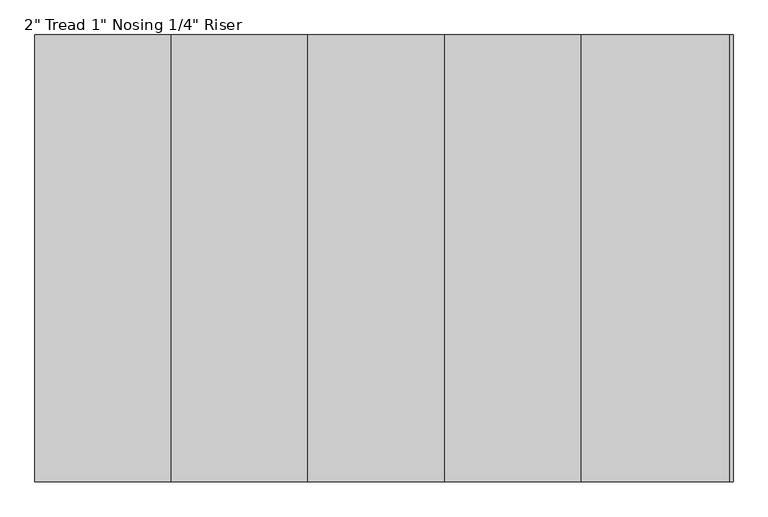
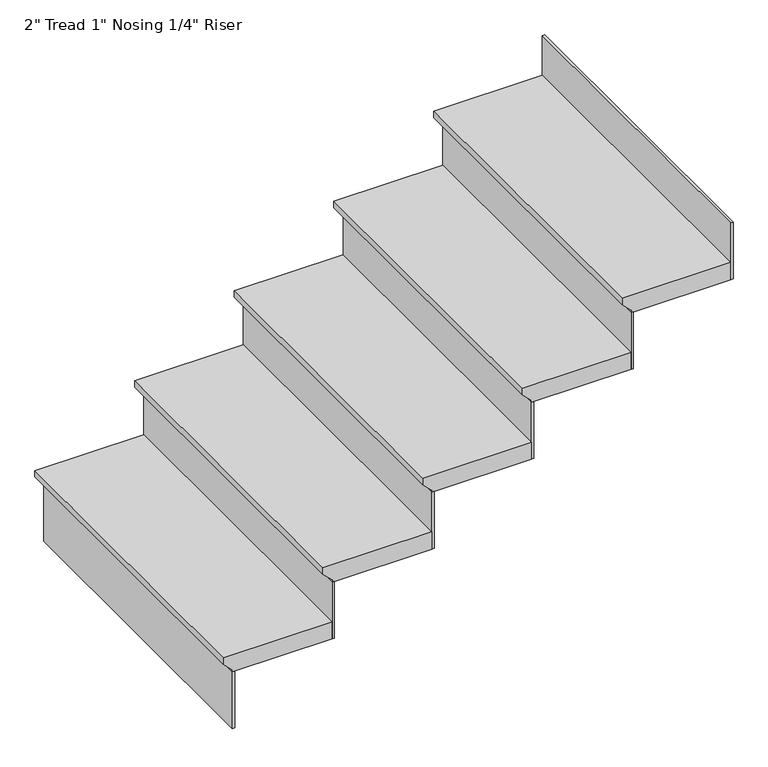
"""IFC4 building model written with IfcOpenShell, lengths in millimetres: stair flight geometry."""

from ifc_helpers import new_model, si_unit, frame, origin, place, context, project, spatial, polyline, outline, extrude, source, transform, mapped, element, save


def stair_flight_cfa6a4ea(model_context):
    return source(origin(), model_context, "Body", "SweptSolid", [
        extrude(outline(polyline([(265553.825, 25477.7840778), (265553.825, 25172.9840778), (265534.775, 25172.9840778), (265509.375, 25198.3840778), (265503.025, 25198.3840778), (265503.025, 25477.7840778), (265553.825, 25477.7840778)])), frame((0.0, 25862.6156612, 0.0), z_axis=(0.0, 1.0, 0.0), x_axis=(0.0, 0.0, 1.0)), (0.0, 0.0, 1.0), 914.4),
        extrude(outline(polyline([(25204.7340778, 25862.6156612), (25198.3840778, 25862.6156612), (25198.3840778, 26777.0156612), (25204.7340778, 26777.0156612), (25204.7340778, 25862.6156612)])), frame((0.0, 0.0, 265334.75), z_axis=(0.0, 0.0, 1.0), x_axis=(1.0, 0.0, 0.0)), (0.0, 0.0, 1.0), 168.275),
        extrude(outline(polyline([(25484.1340778, 25862.6156612), (25477.7840778, 25862.6156612), (25477.7840778, 26777.0156612), (25484.1340778, 26777.0156612), (25484.1340778, 25862.6156612)])), frame((0.0, 0.0, 265503.025), z_axis=(0.0, 0.0, 1.0), x_axis=(1.0, 0.0, 0.0)), (0.0, 0.0, 1.0), 168.275),
        extrude(outline(polyline([(265722.1, 25757.1840778), (265722.1, 25452.3840778), (265703.05, 25452.3840778), (265677.65, 25477.7840778), (265671.3, 25477.7840778), (265671.3, 25757.1840778), (265722.1, 25757.1840778)])), frame((0.0, 25862.6156612, 0.0), z_axis=(0.0, 1.0, 0.0), x_axis=(0.0, 0.0, 1.0)), (0.0, 0.0, 1.0), 914.4),
        extrude(outline(polyline([(25763.5340778, 25862.6156612), (25757.1840778, 25862.6156612), (25757.1840778, 26777.0156612), (25763.5340778, 26777.0156612), (25763.5340778, 25862.6156612)])), frame((0.0, 0.0, 265671.3), z_axis=(0.0, 0.0, 1.0), x_axis=(1.0, 0.0, 0.0)), (0.0, 0.0, 1.0), 168.275),
        extrude(outline(polyline([(265890.375, 26036.5840778), (265890.375, 25731.7840778), (265871.325, 25731.7840778), (265845.925, 25757.1840778), (265839.575, 25757.1840778), (265839.575, 26036.5840778), (265890.375, 26036.5840778)])), frame((0.0, 25862.6156612, 0.0), z_axis=(0.0, 1.0, 0.0), x_axis=(0.0, 0.0, 1.0)), (0.0, 0.0, 1.0), 914.4),
        extrude(outline(polyline([(26042.9340778, 25862.6156612), (26036.5840778, 25862.6156612), (26036.5840778, 26777.0156612), (26042.9340778, 26777.0156612), (26042.9340778, 25862.6156612)])), frame((0.0, 0.0, 265839.575), z_axis=(0.0, 0.0, 1.0), x_axis=(1.0, 0.0, 0.0)), (0.0, 0.0, 1.0), 168.275),
        extrude(outline(polyline([(266058.65, 26315.9840778), (266058.65, 26011.1840778), (266039.6, 26011.1840778), (266014.2, 26036.5840778), (266007.85, 26036.5840778), (266007.85, 26315.9840778), (266058.65, 26315.9840778)])), frame((0.0, 25862.6156612, 0.0), z_axis=(0.0, 1.0, 0.0), x_axis=(0.0, 0.0, 1.0)), (0.0, 0.0, 1.0), 914.4),
        extrude(outline(polyline([(26322.3340778, 25862.6156612), (26315.9840778, 25862.6156612), (26315.9840778, 26777.0156612), (26322.3340778, 26777.0156612), (26322.3340778, 25862.6156612)])), frame((0.0, 0.0, 266007.85), z_axis=(0.0, 0.0, 1.0), x_axis=(1.0, 0.0, 0.0)), (0.0, 0.0, 1.0), 168.275),
        extrude(outline(polyline([(26601.7340778, 25862.6156612), (26595.3840778, 25862.6156612), (26595.3840778, 26777.0156612), (26601.7340778, 26777.0156612), (26601.7340778, 25862.6156612)])), frame((0.0, 0.0, 266176.125), z_axis=(0.0, 0.0, 1.0), x_axis=(1.0, 0.0, 0.0)), (0.0, 0.0, 1.0), 168.275),
        extrude(outline(polyline([(266226.925, 26595.3840778), (266226.925, 26290.5840778), (266207.875, 26290.5840778), (266182.475, 26315.9840778), (266176.125, 26315.9840778), (266176.125, 26595.3840778), (266226.925, 26595.3840778)])), frame((0.0, 25862.6156612, 0.0), z_axis=(0.0, 1.0, 0.0), x_axis=(0.0, 0.0, 1.0)), (0.0, 0.0, 1.0), 914.4),
    ])


if __name__ == "__main__":
    model = new_model("IFC4")
    model_context = context("Model", 3, world=origin())
    ifc_project = project(units=[si_unit("LENGTHUNIT", "METRE", prefix="MILLI")], contexts=[model_context])
    site = spatial("IfcSite", under=ifc_project)
    building = spatial("IfcBuilding", under=site)
    placement = place(None, origin())
    stair_flight_shape = stair_flight_cfa6a4ea(model_context)
    element("IfcStairFlight", 1, ObjectType="2\" Tread 1\" Nosing 1/4\" Riser", at=placement, inside=building, context=model_context, shape_type="MappedRepresentation", body=[
        mapped(stair_flight_shape, transform((0.0, 0.0, 0.0), x_axis=(1.0, 0.0, 0.0), y_axis=(0.0, 1.0, 0.0), z_axis=(0.0, 0.0, 1.0))),
    ])
    save(model, "model.ifc")

# Revit data of these elements
# Element 1 (IfcStairFlight, "2\" Tread 1\" Nosing 1/4\" Riser")
#   Materials on its faces: "SLOTTED WOOD FENCE (THERMALLY MODIFIED WOOD: ARBOR WOOD)\n(EXTERIOR STAIN : PENOFIN VERDE EXT. STAIN - COLOR: CEDAR)"
# Materials
#   "SLOTTED WOOD FENCE (THERMALLY MODIFIED WOOD: ARBOR WOOD)\n(EXTERIOR STAIN : PENOFIN VERDE EXT. STAIN - COLOR: CEDAR)": class "Wood", colour RGB 164 134 123, transparency 0, Description = "Pinus Echinata", Cost = 0
